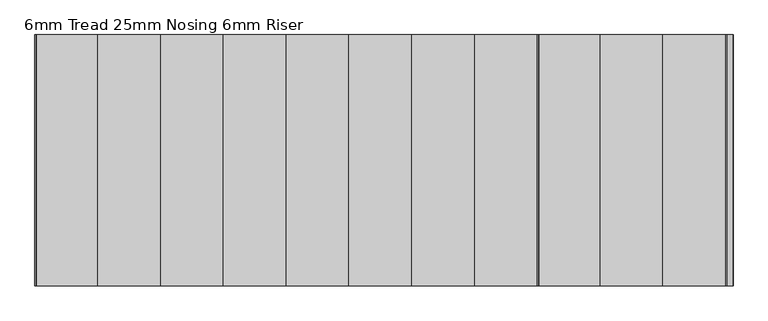
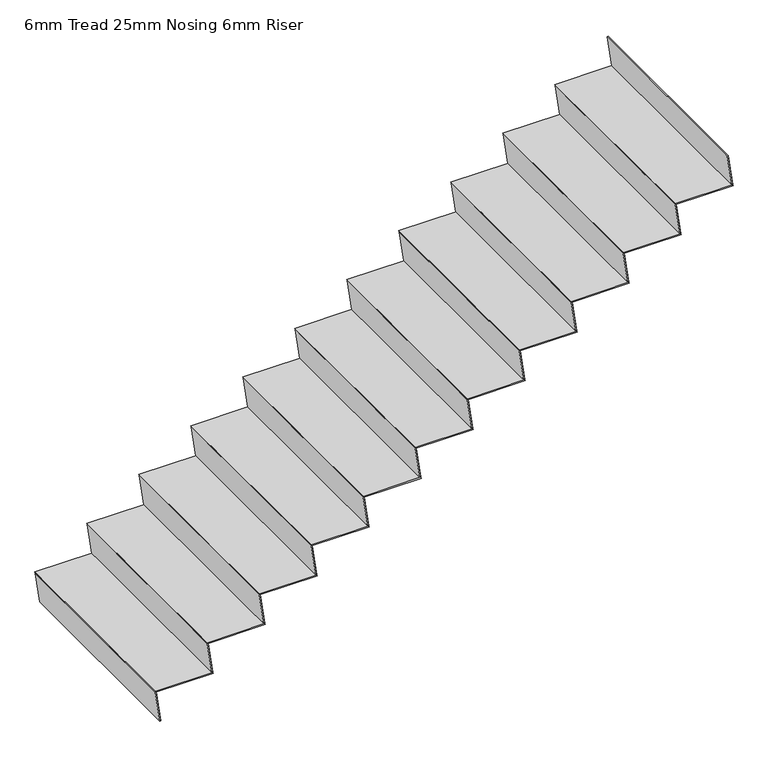
"""IFC4 building model written with IfcOpenShell, lengths in millimetres: stair flight geometry, 6mm Tread 25mm Nosing 6mm Riser."""

from ifc_helpers import new_model, si_unit, origin, place, context, project, spatial, faceted_brep, source, transform, mapped, element, save


def stair_flight_6mm_tread_25mm_nosing_6mm_riser_da47396f(model_context):
    return source(origin(), model_context, "Body", "Brep", [
        faceted_brep([(-16043.9400908, 12030.4345331, 10117.6470588), (-16043.0900908, 12030.4345331, 10111.6470588), (-16043.0900908, 13130.4345331, 10111.6470588), (-16043.9400908, 13130.4345331, 10117.6470588), (-16350.0, 13130.4345331, 10117.6470588), (-16350.0, 12030.4345331, 10117.6470588), (-16349.15, 12030.4345331, 10111.6470588), (-16349.15, 13130.4345331, 10111.6470588)], [[[0, 1, 2, 3]], [[3, 4, 5, 0]], [[2, 1, 6, 7]], [[4, 3, 2, 7]], [[0, 5, 6, 1]], [[5, 4, 7, 6]]]),
        faceted_brep([(-16349.15, 12030.4345331, 10111.6470588), (-16325.0, 12030.4345331, 9941.1764706), (-16318.9400908, 12030.4345331, 9941.1764706), (-16343.0900908, 12030.4345331, 10111.6470588), (-16349.15, 13130.4345331, 10111.6470588), (-16343.0900908, 13130.4345331, 10111.6470588), (-16318.9400908, 13130.4345331, 9941.1764706), (-16325.0, 13130.4345331, 9941.1764706)], [[[0, 1, 2, 3]], [[4, 5, 6, 7]], [[1, 0, 4, 7]], [[2, 1, 7, 6]], [[3, 2, 6, 5]], [[0, 3, 5, 4]]]),
        faceted_brep([(-16074.15, 12030.4345331, 10288.1176471), (-16050.0, 12030.4345331, 10117.6470588), (-16043.9400908, 12030.4345331, 10117.6470588), (-16068.0900908, 12030.4345331, 10288.1176471), (-16074.15, 13130.4345331, 10288.1176471), (-16068.0900908, 13130.4345331, 10288.1176471), (-16043.9400908, 13130.4345331, 10117.6470588), (-16050.0, 13130.4345331, 10117.6470588)], [[[0, 1, 2, 3]], [[4, 5, 6, 7]], [[1, 0, 4, 7]], [[2, 1, 7, 6]], [[3, 2, 6, 5]], [[0, 3, 5, 4]]]),
        faceted_brep([(-15768.9400908, 13130.4345331, 10294.1176471), (-16075.0, 13130.4345331, 10294.1176471), (-16075.0, 12030.4345331, 10294.1176471), (-15768.9400908, 12030.4345331, 10294.1176471), (-15768.0900908, 13130.4345331, 10288.1176471), (-15768.0900908, 12030.4345331, 10288.1176471), (-16074.15, 12030.4345331, 10288.1176471), (-16074.15, 13130.4345331, 10288.1176471)], [[[0, 1, 2, 3]], [[4, 5, 6, 7]], [[1, 0, 4, 7]], [[3, 2, 6, 5]], [[3, 5, 4, 0]], [[2, 1, 7, 6]]]),
        faceted_brep([(-15799.15, 12030.4345331, 10464.5882353), (-15775.0, 12030.4345331, 10294.1176471), (-15768.9400908, 12030.4345331, 10294.1176471), (-15793.0900908, 12030.4345331, 10464.5882353), (-15799.15, 13130.4345331, 10464.5882353), (-15793.0900908, 13130.4345331, 10464.5882353), (-15768.9400908, 13130.4345331, 10294.1176471), (-15775.0, 13130.4345331, 10294.1176471)], [[[0, 1, 2, 3]], [[4, 5, 6, 7]], [[1, 0, 4, 7]], [[2, 1, 7, 6]], [[3, 2, 6, 5]], [[0, 3, 5, 4]]]),
        faceted_brep([(-15493.9400908, 13130.4345331, 10470.5882353), (-15800.0, 13130.4345331, 10470.5882353), (-15800.0, 12030.4345331, 10470.5882353), (-15493.9400908, 12030.4345331, 10470.5882353), (-15493.0900908, 13130.4345331, 10464.5882353), (-15493.0900908, 12030.4345331, 10464.5882353), (-15799.15, 12030.4345331, 10464.5882353), (-15799.15, 13130.4345331, 10464.5882353)], [[[0, 1, 2, 3]], [[4, 5, 6, 7]], [[1, 0, 4, 7]], [[3, 2, 6, 5]], [[3, 5, 4, 0]], [[2, 1, 7, 6]]]),
        faceted_brep([(-15524.15, 12030.4345331, 10641.0588235), (-15500.0, 12030.4345331, 10470.5882353), (-15493.9400908, 12030.4345331, 10470.5882353), (-15518.0900908, 12030.4345331, 10641.0588235), (-15524.15, 13130.4345331, 10641.0588235), (-15518.0900908, 13130.4345331, 10641.0588235), (-15493.9400908, 13130.4345331, 10470.5882353), (-15500.0, 13130.4345331, 10470.5882353)], [[[0, 1, 2, 3]], [[4, 5, 6, 7]], [[1, 0, 4, 7]], [[2, 1, 7, 6]], [[3, 2, 6, 5]], [[0, 3, 5, 4]]]),
        faceted_brep([(-15218.9400908, 13130.4345331, 10647.0588235), (-15525.0, 13130.4345331, 10647.0588235), (-15525.0, 12030.4345331, 10647.0588235), (-15218.9400908, 12030.4345331, 10647.0588235), (-15218.0900908, 13130.4345331, 10641.0588235), (-15218.0900908, 12030.4345331, 10641.0588235), (-15524.15, 12030.4345331, 10641.0588235), (-15524.15, 13130.4345331, 10641.0588235)], [[[0, 1, 2, 3]], [[4, 5, 6, 7]], [[1, 0, 4, 7]], [[3, 2, 6, 5]], [[3, 5, 4, 0]], [[2, 1, 7, 6]]]),
        faceted_brep([(-15249.15, 12030.4345331, 10817.5294118), (-15225.0, 12030.4345331, 10647.0588235), (-15218.9400908, 12030.4345331, 10647.0588235), (-15243.0900908, 12030.4345331, 10817.5294118), (-15249.15, 13130.4345331, 10817.5294118), (-15243.0900908, 13130.4345331, 10817.5294118), (-15218.9400908, 13130.4345331, 10647.0588235), (-15225.0, 13130.4345331, 10647.0588235)], [[[0, 1, 2, 3]], [[4, 5, 6, 7]], [[1, 0, 4, 7]], [[2, 1, 7, 6]], [[3, 2, 6, 5]], [[0, 3, 5, 4]]]),
        faceted_brep([(-14943.9400908, 13130.4345331, 10823.5294118), (-15250.0, 13130.4345331, 10823.5294118), (-15250.0, 12030.4345331, 10823.5294118), (-14943.9400908, 12030.4345331, 10823.5294118), (-14943.0900908, 13130.4345331, 10817.5294118), (-14943.0900908, 12030.4345331, 10817.5294118), (-15249.15, 12030.4345331, 10817.5294118), (-15249.15, 13130.4345331, 10817.5294118)], [[[0, 1, 2, 3]], [[4, 5, 6, 7]], [[1, 0, 4, 7]], [[3, 2, 6, 5]], [[3, 5, 4, 0]], [[2, 1, 7, 6]]]),
        faceted_brep([(-14974.15, 12030.4345331, 10994.0), (-14950.0, 12030.4345331, 10823.5294118), (-14943.9400908, 12030.4345331, 10823.5294118), (-14968.0900908, 12030.4345331, 10994.0), (-14974.15, 13130.4345331, 10994.0), (-14968.0900908, 13130.4345331, 10994.0), (-14943.9400908, 13130.4345331, 10823.5294118), (-14950.0, 13130.4345331, 10823.5294118)], [[[0, 1, 2, 3]], [[4, 5, 6, 7]], [[1, 0, 4, 7]], [[2, 1, 7, 6]], [[3, 2, 6, 5]], [[0, 3, 5, 4]]]),
        faceted_brep([(-14668.9400908, 13130.4345331, 11000.0), (-14975.0, 13130.4345331, 11000.0), (-14975.0, 12030.4345331, 11000.0), (-14668.9400908, 12030.4345331, 11000.0), (-14668.0900908, 13130.4345331, 10994.0), (-14668.0900908, 12030.4345331, 10994.0), (-14974.15, 12030.4345331, 10994.0), (-14974.15, 13130.4345331, 10994.0)], [[[0, 1, 2, 3]], [[4, 5, 6, 7]], [[1, 0, 4, 7]], [[3, 2, 6, 5]], [[3, 5, 4, 0]], [[2, 1, 7, 6]]]),
        faceted_brep([(-14699.15, 12030.4345331, 11170.4705882), (-14675.0, 12030.4345331, 11000.0), (-14668.9400908, 12030.4345331, 11000.0), (-14693.0900908, 12030.4345331, 11170.4705882), (-14699.15, 13130.4345331, 11170.4705882), (-14693.0900908, 13130.4345331, 11170.4705882), (-14668.9400908, 13130.4345331, 11000.0), (-14675.0, 13130.4345331, 11000.0)], [[[0, 1, 2, 3]], [[4, 5, 6, 7]], [[1, 0, 4, 7]], [[2, 1, 7, 6]], [[3, 2, 6, 5]], [[0, 3, 5, 4]]]),
        faceted_brep([(-14393.9400908, 13130.4345331, 11176.4705882), (-14700.0, 13130.4345331, 11176.4705882), (-14700.0, 12030.4345331, 11176.4705882), (-14393.9400908, 12030.4345331, 11176.4705882), (-14393.0900908, 13130.4345331, 11170.4705882), (-14393.0900908, 12030.4345331, 11170.4705882), (-14699.15, 12030.4345331, 11170.4705882), (-14699.15, 13130.4345331, 11170.4705882)], [[[0, 1, 2, 3]], [[4, 5, 6, 7]], [[1, 0, 4, 7]], [[3, 2, 6, 5]], [[3, 5, 4, 0]], [[2, 1, 7, 6]]]),
        faceted_brep([(-14424.15, 12030.4345331, 11346.9411765), (-14400.0, 12030.4345331, 11176.4705882), (-14393.9400908, 12030.4345331, 11176.4705882), (-14418.0900908, 12030.4345331, 11346.9411765), (-14424.15, 13130.4345331, 11346.9411765), (-14418.0900908, 13130.4345331, 11346.9411765), (-14393.9400908, 13130.4345331, 11176.4705882), (-14400.0, 13130.4345331, 11176.4705882)], [[[0, 1, 2, 3]], [[4, 5, 6, 7]], [[1, 0, 4, 7]], [[2, 1, 7, 6]], [[3, 2, 6, 5]], [[0, 3, 5, 4]]]),
        faceted_brep([(-14118.9400908, 13130.4345331, 11352.9411765), (-14425.0, 13130.4345331, 11352.9411765), (-14425.0, 12030.4345331, 11352.9411765), (-14118.9400908, 12030.4345331, 11352.9411765), (-14118.0900908, 13130.4345331, 11346.9411765), (-14118.0900908, 12030.4345331, 11346.9411765), (-14424.15, 12030.4345331, 11346.9411765), (-14424.15, 13130.4345331, 11346.9411765)], [[[0, 1, 2, 3]], [[4, 5, 6, 7]], [[1, 0, 4, 7]], [[3, 2, 6, 5]], [[3, 5, 4, 0]], [[2, 1, 7, 6]]]),
        faceted_brep([(-14149.15, 12030.4345331, 11523.4117647), (-14125.0, 12030.4345331, 11352.9411765), (-14118.9400908, 12030.4345331, 11352.9411765), (-14143.0900908, 12030.4345331, 11523.4117647), (-14149.15, 13130.4345331, 11523.4117647), (-14143.0900908, 13130.4345331, 11523.4117647), (-14118.9400908, 13130.4345331, 11352.9411765), (-14125.0, 13130.4345331, 11352.9411765)], [[[0, 1, 2, 3]], [[4, 5, 6, 7]], [[1, 0, 4, 7]], [[2, 1, 7, 6]], [[3, 2, 6, 5]], [[0, 3, 5, 4]]]),
        faceted_brep([(-13843.9400908, 13130.4345331, 11529.4117647), (-14150.0, 13130.4345331, 11529.4117647), (-14150.0, 12030.4345331, 11529.4117647), (-13843.9400908, 12030.4345331, 11529.4117647), (-13843.0900908, 13130.4345331, 11523.4117647), (-13843.0900908, 12030.4345331, 11523.4117647), (-14149.15, 12030.4345331, 11523.4117647), (-14149.15, 13130.4345331, 11523.4117647)], [[[0, 1, 2, 3]], [[4, 5, 6, 7]], [[1, 0, 4, 7]], [[3, 2, 6, 5]], [[3, 5, 4, 0]], [[2, 1, 7, 6]]]),
        faceted_brep([(-13874.15, 12030.4345331, 11699.8823529), (-13850.0, 12030.4345331, 11529.4117647), (-13843.9400908, 12030.4345331, 11529.4117647), (-13868.0900908, 12030.4345331, 11699.8823529), (-13874.15, 13130.4345331, 11699.8823529), (-13868.0900908, 13130.4345331, 11699.8823529), (-13843.9400908, 13130.4345331, 11529.4117647), (-13850.0, 13130.4345331, 11529.4117647)], [[[0, 1, 2, 3]], [[4, 5, 6, 7]], [[1, 0, 4, 7]], [[2, 1, 7, 6]], [[3, 2, 6, 5]], [[0, 3, 5, 4]]]),
        faceted_brep([(-13568.9400908, 13130.4345331, 11705.8823529), (-13875.0, 13130.4345331, 11705.8823529), (-13875.0, 12030.4345331, 11705.8823529), (-13568.9400908, 12030.4345331, 11705.8823529), (-13568.0900908, 13130.4345331, 11699.8823529), (-13568.0900908, 12030.4345331, 11699.8823529), (-13874.15, 12030.4345331, 11699.8823529), (-13874.15, 13130.4345331, 11699.8823529)], [[[0, 1, 2, 3]], [[4, 5, 6, 7]], [[1, 0, 4, 7]], [[3, 2, 6, 5]], [[3, 5, 4, 0]], [[2, 1, 7, 6]]]),
        faceted_brep([(-13324.15, 12030.4345331, 12052.8235294), (-13300.0, 12030.4345331, 11882.3529412), (-13293.9400908, 12030.4345331, 11882.3529412), (-13318.0900908, 12030.4345331, 12052.8235294), (-13324.15, 13130.4345331, 12052.8235294), (-13318.0900908, 13130.4345331, 12052.8235294), (-13293.9400908, 13130.4345331, 11882.3529412), (-13300.0, 13130.4345331, 11882.3529412)], [[[0, 1, 2, 3]], [[4, 5, 6, 7]], [[1, 0, 4, 7]], [[2, 1, 7, 6]], [[3, 2, 6, 5]], [[0, 3, 5, 4]]]),
        faceted_brep([(-13599.15, 12030.4345331, 11876.3529412), (-13575.0, 12030.4345331, 11705.8823529), (-13568.9400908, 12030.4345331, 11705.8823529), (-13593.0900908, 12030.4345331, 11876.3529412), (-13599.15, 13130.4345331, 11876.3529412), (-13593.0900908, 13130.4345331, 11876.3529412), (-13568.9400908, 13130.4345331, 11705.8823529), (-13575.0, 13130.4345331, 11705.8823529)], [[[0, 1, 2, 3]], [[4, 5, 6, 7]], [[1, 0, 4, 7]], [[2, 1, 7, 6]], [[3, 2, 6, 5]], [[0, 3, 5, 4]]]),
        faceted_brep([(-13293.9400908, 13130.4345331, 11882.3529412), (-13325.0, 13130.4345331, 11882.3529412), (-13600.0, 13130.4345331, 11882.3529412), (-13600.0, 12030.4345331, 11882.3529412), (-13293.9400908, 12030.4345331, 11882.3529412), (-13293.0900908, 13130.4345331, 11876.3529412), (-13293.0900908, 12030.4345331, 11876.3529412), (-13599.15, 12030.4345331, 11876.3529412), (-13599.15, 13130.4345331, 11876.3529412), (-13325.0, 13130.4345331, 11876.3529412)], [[[0, 1, 2, 3, 4]], [[5, 6, 7, 8, 9]], [[1, 0, 5, 9]], [[2, 1, 9, 8]], [[4, 3, 7, 6]], [[4, 6, 5, 0]], [[3, 2, 8, 7]]]),
    ])


if __name__ == "__main__":
    model = new_model("IFC4")
    model_context = context("Model", 3, world=origin())
    ifc_project = project(units=[si_unit("LENGTHUNIT", "METRE", prefix="MILLI")], contexts=[model_context])
    site = spatial("IfcSite", under=ifc_project)
    building = spatial("IfcBuilding", under=site)
    placement = place(None, origin())
    stair_flight_6mm_tread_25mm_nosing_6mm_riser_shape = stair_flight_6mm_tread_25mm_nosing_6mm_riser_da47396f(model_context)
    element("IfcStairFlight", 1, ObjectType="6mm Tread 25mm Nosing 6mm Riser", at=placement, inside=building, context=model_context, shape_type="MappedRepresentation", body=[
        mapped(stair_flight_6mm_tread_25mm_nosing_6mm_riser_shape, transform((0.0, 0.0, 0.0), x_axis=(1.0, 0.0, 0.0), y_axis=(0.0, 1.0, 0.0), z_axis=(0.0, 0.0, 1.0))),
    ])
    save(model, "model.ifc")

# Revit data of these elements
# Element 1 (IfcStairFlight, "6mm Tread 25mm Nosing 6mm Riser")
#   Materials on its faces: "Steel, Paint Finish, Dark Gray"
# Materials
#   "Steel, Paint Finish, Dark Gray": class "Metal", colour RGB 89 89 89, transparency 0, Description = "Steel, paint finish, dark gray, glossy", Cost = 0
